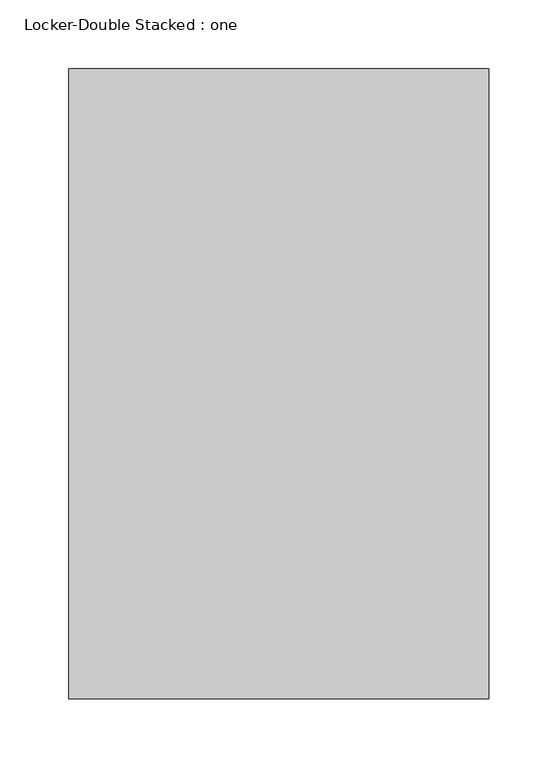
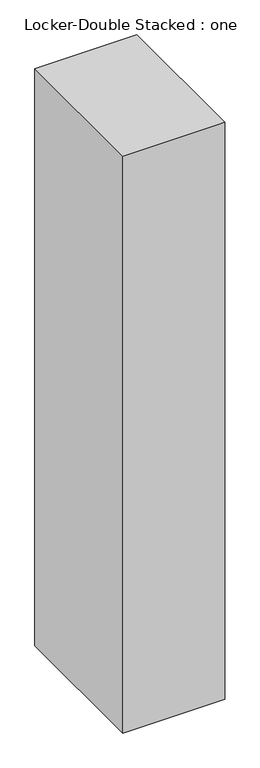
"""IFC4 building model written with IfcOpenShell, lengths in millimetres: furniture geometry, Locker-Double Stacked : one."""

from ifc_helpers import new_model, si_unit, origin, place, context, project, spatial, faceted_brep, source, transform, mapped, element, save


def locker_double_stacked_one_7b1cf9e5(model_context):
    return source(origin(), model_context, "Body", "Brep", [
        faceted_brep([(152.4, 228.6, 1828.8), (-152.4, 228.6, 1828.8), (-152.4, -228.6, 1828.8), (152.4, -228.6, 1828.8), (152.4, 228.6, 0.0), (152.4, -228.6, 0.0), (-152.4, -228.6, 0.0), (-152.4, 228.6, 0.0), (127.0, 228.6, 889.0), (-127.0, 228.6, 889.0), (-127.0, 228.6, 76.2), (127.0, 228.6, 76.2), (-127.0, 228.6, 1752.6), (-127.0, 228.6, 939.8), (127.0, 228.6, 939.8), (127.0, 228.6, 1752.6), (127.0, 222.25, 76.2), (-127.0, 222.25, 76.2), (-127.0, 222.25, 889.0), (127.0, 222.25, 889.0), (127.0, 222.25, 1752.6), (127.0, 222.25, 939.8), (-127.0, 222.25, 939.8), (-127.0, 222.25, 1752.6)], [[[0, 1, 2, 3]], [[4, 5, 6, 7]], [[3, 5, 4, 0]], [[2, 6, 5, 3]], [[1, 7, 6, 2]], [[0, 4, 7, 1], [8, 9, 10, 11], [12, 13, 14, 15]], [[16, 17, 18, 19]], [[19, 8, 11, 16]], [[18, 9, 8, 19]], [[17, 10, 9, 18]], [[16, 11, 10, 17]], [[20, 21, 22, 23]], [[23, 12, 15, 20]], [[22, 13, 12, 23]], [[21, 14, 13, 22]], [[20, 15, 14, 21]]]),
    ])


if __name__ == "__main__":
    model = new_model("IFC4")
    model_context = context("Model", 3, world=origin())
    ifc_project = project(units=[si_unit("LENGTHUNIT", "METRE", prefix="MILLI")], contexts=[model_context])
    site = spatial("IfcSite", under=ifc_project)
    building = spatial("IfcBuilding", under=site)
    placement = place(None, origin())
    locker_double_stacked_one_shape = locker_double_stacked_one_7b1cf9e5(model_context)
    element("IfcFurniture", 1, ObjectType="Locker-Double Stacked : one", at=placement, inside=building, context=model_context, shape_type="MappedRepresentation", body=[
        mapped(locker_double_stacked_one_shape, transform((0.0, 0.0, 0.0), x_axis=(1.0, 0.0, 0.0), y_axis=(0.0, 1.0, 0.0), z_axis=(0.0, 0.0, 1.0))),
    ])
    save(model, "model.ifc")

# Revit data of these elements
# Type "Locker-Double Stacked : one"
#   Keynote = "M10511300.01"
#   Assembly Code = "E2010"
#   Depth = 1' - 6"
#   Height = 6' - 0"
#   Width = 1' - 0"
#   Material = Metal - Paint Finish - Dark Gray, Matte
# Element 1 (IfcFurniture, "Locker-Double Stacked : one")
#   Materials on its faces: "Metal - Paint Finish - Dark Gray, Matte"
# Materials
#   "Metal - Paint Finish - Dark Gray, Matte": class "Metal", colour RGB 98 98 98, transparency 0
